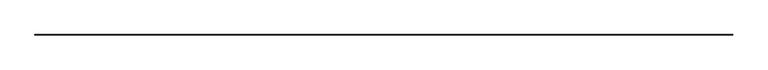
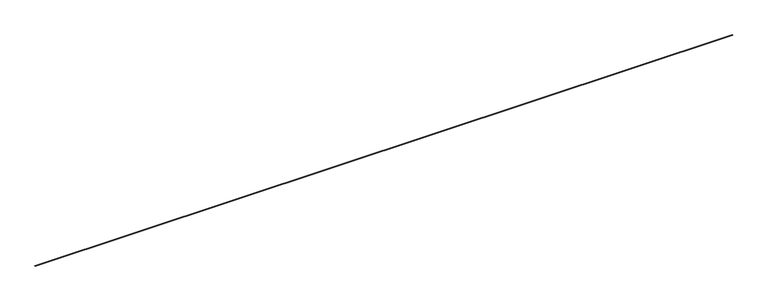
"""IFC4 building model written with IfcOpenShell, lengths in millimetres: proxy geometry, Inner panel:Inner panel:1:Inner panel:1 : Inner panel:Inner panel:300324:2:Inner panel:1:Inner panel:1 : Inner panel:Inner panel:300324:2 : Inner panel:Inner panel:1:Inner panel:1 : Inner panel:Inner panel:300324:300043:19 : Inner panel:Inner panel:1:Inner panel:1 : Inner panel:Inner panel:300324:2:Inner panel:1:Inner panel:1 : Inner panel:Inner panel:300324:2 : Inner panel:Inner panel:1:Inner panel:1 : Inner panel:Inner panel:300324:300043:308120."""

from ifc_helpers import new_model, si_unit, frame, origin, place, context, project, spatial, polyline, outline, extrude, source, transform, mapped, element, save


def generic_models_b6840ea7(model_context):
    return source(origin(), model_context, "Body", "SweptSolid", [
        extrude(outline(polyline([(-568966.8701052, 8733.0533659), (-568968.4562289, 8771.1203359), (-568930.3892588, 8772.7064597), (-568928.8031351, 8734.6394896), (-568966.8701052, 8733.0533659)]), holes=[polyline([(-568964.5900523, 8735.5316842), (-568931.2814535, 8736.9195425), (-568932.6693117, 8770.2281413), (-568965.9779106, 8768.8402831), (-568964.5900523, 8735.5316842)])]), frame((579104.5117239, 0.0, 0.0), z_axis=(1.0, 0.0, 0.0), x_axis=(0.0, 1.0, 0.0)), (0.0, 0.0, 1.0), 88442.8),
    ])


if __name__ == "__main__":
    model = new_model("IFC4")
    model_context = context("Model", 3, world=origin())
    ifc_project = project(units=[si_unit("LENGTHUNIT", "METRE", prefix="MILLI")], contexts=[model_context])
    site = spatial("IfcSite", under=ifc_project)
    building = spatial("IfcBuilding", under=site)
    placement = place(None, origin())
    generic_models_shape = generic_models_b6840ea7(model_context)
    element("IfcBuildingElementProxy", 1, Name="Inner panel:Inner panel:1:Inner panel:1 : Inner panel:Inner panel:300324:2:Inner panel:1:Inner panel:1 : Inner panel:Inner panel:300324:2 : Inner panel:Inner panel:1:Inner panel:1 : Inner panel:Inner panel:300324:300043:19 : Inner panel:Inner panel:1:Inner panel:1 : Inner panel:Inner panel:300324:2:Inner panel:1:Inner panel:1 : Inner panel:Inner panel:300324:2 : Inner panel:Inner panel:1:Inner panel:1 : Inner panel:Inner panel:300324:300043:308120", ObjectType="Inner panel:Inner panel:1:Inner panel:1 : Inner panel:Inner panel:300324:2:Inner panel:1:Inner panel:1 : Inner panel:Inner panel:300324:2 : Inner panel:Inner panel:1:Inner panel:1 : Inner panel:Inner panel:300324:300043:19 : Inner panel:Inner panel:1:Inner panel:1 : Inner panel:Inner panel:300324:2:Inner panel:1:Inner panel:1 : Inner panel:Inner panel:300324:2 : Inner panel:Inner panel:1:Inner panel:1 : Inner panel:Inner panel:300324:300043:308120", at=placement, inside=building, context=model_context, shape_type="MappedRepresentation", body=[
        mapped(generic_models_shape, transform((0.0, 0.0, 0.0), x_axis=(1.0, 0.0, 0.0), y_axis=(0.0, 1.0, 0.0), z_axis=(0.0, 0.0, 1.0))),
    ])
    save(model, "model.ifc")

# Revit data of these elements
# Type "Inner panel:Inner panel:1:Inner panel:1 : Inner panel:Inner panel:300324:2:Inner panel:1:Inner panel:1 : Inner panel:Inner panel:300324:2 : Inner panel:Inner panel:1:Inner panel:1 : Inner panel:Inner panel:300324:300043:19 : Inner panel:Inner panel:1:Inner panel:1 : Inner panel:Inner panel:300324:2:Inner panel:1:Inner panel:1 : Inner panel:Inner panel:300324:2 : Inner panel:Inner panel:1:Inner panel:1 : Inner panel:Inner panel:300324:300043:308120"
#   NameOverride = "Inner panel:Inner panel:1:Inner panel:1 : Inner panel:Inner panel:300324:2:Inner panel:1:Inner panel:1 : Inner panel:Inner panel:300324:2 : Inner panel:Inner panel:1:Inner panel:1 : Inner panel:Inner panel:300324:300043:308120"
#   ObjectTypeOverride = "Inner panel:1:Inner panel:1 : Inner panel:Inner panel:300324:2 : Inner panel:Inner panel:1:Inner panel:1 : Inner panel:Inner panel:300324:300043"
#   Reference = "Inner panel"
#   Tag = "308120"
# Element 1 (IfcBuildingElementProxy, "Inner panel:Inner panel:1:Inner panel:1 : Inner panel:Inner panel:300324:2:Inner panel:1:Inner panel:1 : Inner panel:Inner panel:300324:2 : Inner panel:Inner panel:1:Inner panel:1 : Inner panel:Inner panel:300324:300043:19 : Inner panel:Inner panel:1:Inner panel:1 : Inner panel:Inner panel:300324:2:Inner panel:1:Inner panel:1 : Inner panel:Inner panel:300324:2 : Inner panel:Inner panel:1:Inner panel:1 : Inner panel:Inner panel:300324:300043:308120")
#   Materials on its faces: "1 1/2\" X 1 1/2\" x 1/8\" ALUM. TUBE (6061-T6) - (2) #16 WOOD SCREWS WITH 2.5\" EMBED AT EACH GLULAM - (1) SCREW AT ENDS"
# Materials
#   "1 1/2\" X 1 1/2\" x 1/8\" ALUM. TUBE (6061-T6) - (2) #16 WOOD SCREWS WITH 2.5\" EMBED AT EACH GLULAM - (1) SCREW AT ENDS": class "Unassigned", colour RGB 202 201 200, transparency 0, Cost = 0
